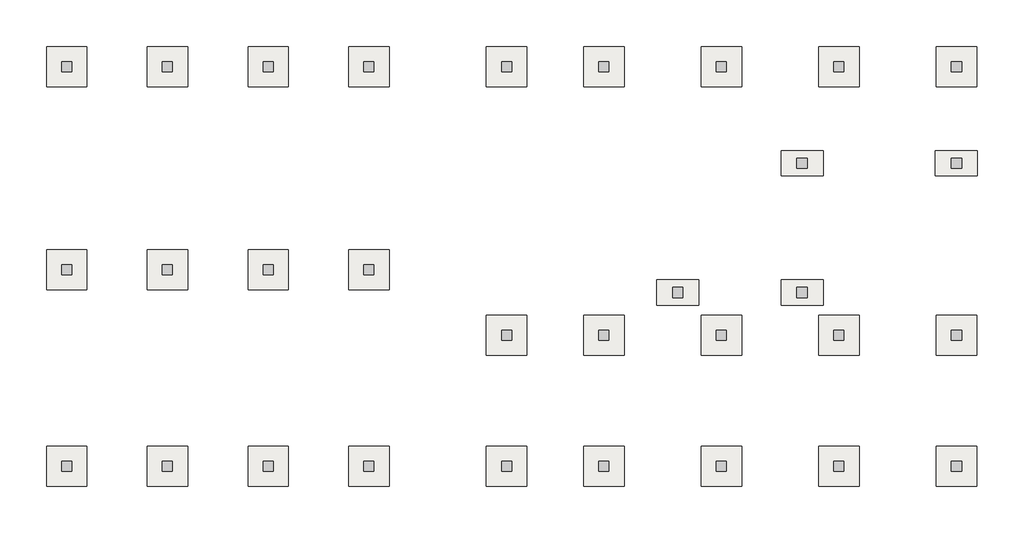
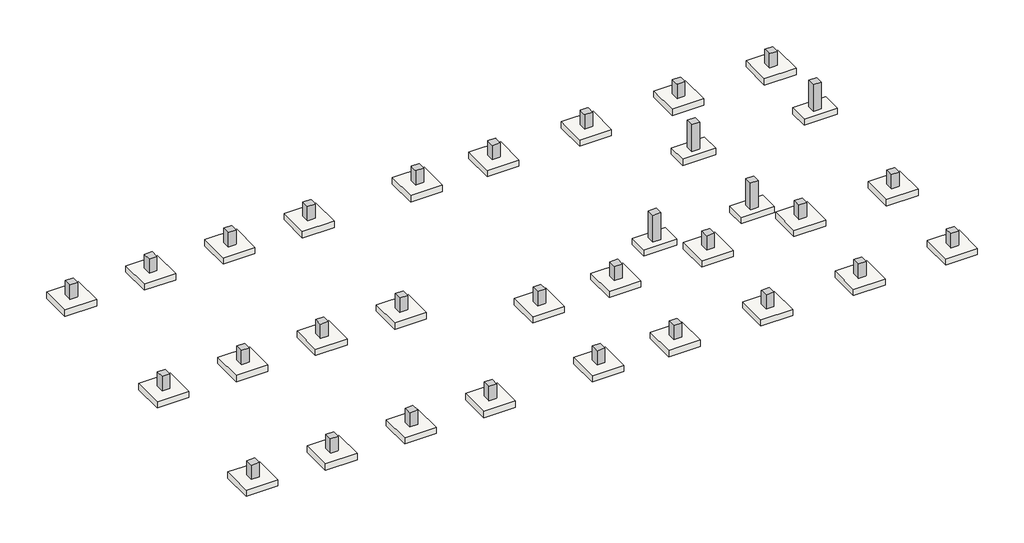
# Not in any storey: 31 columns, 31 slabs.
"""IFC4 building model written with IfcOpenShell, lengths in millimetres."""

import ifcopenshell
import ifcopenshell.guid

model = None  # the IFC model being written
_history = None  # IfcOwnerHistory: only IFC2X3 demands one
_inside = {}  # id of a spatial element -> (the spatial element, [elements in it])
_under = {}  # id of a project, library or spatial element -> (it, [spatial elements below it])
_declared = {}  # id of a project -> (the project, [libraries it declares])
_typed = {}  # id of a type object -> (the type object, [elements of that type])
_made_of = {}  # id of a material, layer set ... -> (it, [elements and type objects made of it])


def new_model(schema):
    """Start an empty IFC model of exactly this schema.

    Asked for "IFC4X3", IfcOpenShell would pick the latest addendum, in which some entities
    have other attributes; the version numbers below select the first issue.
    IFC2X3 requires an IfcOwnerHistory on every rooted entity: one is made here for all.
    """
    global model, _history
    if schema == "IFC4X3":
        model = ifcopenshell.file(schema_version=(4, 3, 0, 0))
    else:
        model = ifcopenshell.file(schema=schema)
    _inside.clear()
    _under.clear()
    _declared.clear()
    _typed.clear()
    _made_of.clear()
    _history = None
    if model.schema == "IFC2X3":
        org = make("IfcOrganization", Name="unknown")
        user = make(
            "IfcPersonAndOrganization",
            ThePerson=make("IfcPerson", FamilyName="unknown"),
            TheOrganization=org,
        )
        app = make(
            "IfcApplication",
            ApplicationDeveloper=org,
            Version="unknown",
            ApplicationFullName="unknown",
            ApplicationIdentifier="unknown",
        )
        _history = make(
            "IfcOwnerHistory",
            OwningUser=user,
            OwningApplication=app,
            ChangeAction="ADDED",
            CreationDate=0,
        )
    return model


def make(cls, **values):
    """One entity of the class cls with the attributes given. An attribute that is None is left unset."""
    return model.create_entity(
        cls, **{name: value for name, value in values.items() if value is not None}
    )


def rooted(cls, **values):
    """An entity with a GlobalId (a new one), such as an element, a storey or a relation."""
    return make(cls, GlobalId=ifcopenshell.guid.new(), OwnerHistory=_history, **values)


def si_unit(unit_type, name, prefix=None):
    """IfcSIUnit, for example si_unit("LENGTHUNIT", "METRE", prefix="MILLI")."""
    return make("IfcSIUnit", UnitType=unit_type, Prefix=prefix, Name=name)


def assignment(units):
    """IfcUnitAssignment: the units of a project."""
    return None if units is None else make("IfcUnitAssignment", Units=units)


def point(xyz):
    """IfcCartesianPoint."""
    return None if xyz is None else make("IfcCartesianPoint", Coordinates=xyz)


def direction(xyz):
    """IfcDirection."""
    return None if xyz is None else make("IfcDirection", DirectionRatios=xyz)


def frame(location, z_axis=None, x_axis=None):
    """IfcAxis2Placement3D, a coordinate frame: its origin and axes. An axis left out is left unset."""
    return make(
        "IfcAxis2Placement3D",
        Location=point(location),
        Axis=direction(z_axis),
        RefDirection=direction(x_axis),
    )


def origin():
    """The frame at (0, 0, 0) with its axes left unset."""
    return frame((0.0, 0.0, 0.0))


def place(relative_to, where):
    """IfcLocalPlacement: puts the frame where relative to a parent placement (None: the world)."""
    return make(
        "IfcLocalPlacement", PlacementRelTo=relative_to, RelativePlacement=where
    )


def context(
    kind, dimensions, precision=None, world=None, true_north=None, identifier=None
):
    """IfcGeometricRepresentationContext, for example the 3D "Model" context."""
    return make(
        "IfcGeometricRepresentationContext",
        ContextIdentifier=identifier,
        ContextType=kind,
        CoordinateSpaceDimension=dimensions,
        Precision=precision,
        WorldCoordinateSystem=world,
        TrueNorth=true_north,
    )


def project(units=None, contexts=None):
    """IfcProject with its units and contexts."""
    return rooted(
        "IfcProject",
        Name="project",
        RepresentationContexts=contexts,
        UnitsInContext=assignment(units),
    )


def spatial(cls, under=None, at=None, **own):
    """A site, building, storey or space (cls), placed at a placement, below another one or the project."""
    s = rooted(cls, ObjectPlacement=at, **own)
    if under is not None:
        _under.setdefault(under.id(), (under, []))[1].append(s)
    return s


def polyline(points):
    """IfcPolyline through the points."""
    return make("IfcPolyline", Points=[point(p) for p in points])


def outline(outer, holes=None, kind="AREA"):
    """IfcArbitraryClosedProfileDef: a profile drawn as a closed curve; with holes, ...WithVoids."""
    if holes is None:
        return make("IfcArbitraryClosedProfileDef", ProfileType=kind, OuterCurve=outer)
    return make(
        "IfcArbitraryProfileDefWithVoids",
        ProfileType=kind,
        OuterCurve=outer,
        InnerCurves=holes,
    )


def extrude(swept, where, along, depth):
    """IfcExtrudedAreaSolid: the profile swept, set in the frame where, extruded along a direction by depth."""
    return make(
        "IfcExtrudedAreaSolid",
        SweptArea=swept,
        Position=where,
        ExtrudedDirection=direction(along),
        Depth=depth,
    )


def faces_of(points, faces, orient=None, outer=None):
    """IfcFace entities. A face is a list of loops; a loop is a list of indices into points, from 0.

    orient and outer hold one flag for each loop. By default every Orientation is true, the
    first loop of a face is its IfcFaceOuterBound and the others are IfcFaceBound.
    """
    made = []
    for i, loops in enumerate(faces):
        bounds = []
        for j, loop in enumerate(loops):
            is_outer = j == 0 if outer is None else outer[i][j]
            bounds.append(
                make(
                    "IfcFaceOuterBound" if is_outer else "IfcFaceBound",
                    Bound=make("IfcPolyLoop", Polygon=[points[k] for k in loop]),
                    Orientation=True if orient is None else orient[i][j],
                )
            )
        made.append(make("IfcFace", Bounds=bounds))
    return made


def faceted_brep(points, faces, orient=None, outer=None, voids=None):
    """IfcFacetedBrep: a solid bounded by flat faces; with voids (closed shells), ...WithVoids."""
    shared = [point(p) for p in points]
    hull = make("IfcClosedShell", CfsFaces=faces_of(shared, faces, orient, outer))
    if voids is None:
        return make("IfcFacetedBrep", Outer=hull)
    return make(
        "IfcFacetedBrepWithVoids",
        Outer=hull,
        Voids=[
            make(cls, CfsFaces=faces_of(shared, fs, o, b)) for cls, fs, o, b in voids
        ],
    )


def shape(context_of_items, identifier, shape_type, items):
    """IfcShapeRepresentation: the items that make up one representation, for example the "Body"."""
    return make(
        "IfcShapeRepresentation",
        ContextOfItems=context_of_items,
        RepresentationIdentifier=identifier,
        RepresentationType=shape_type,
        Items=items,
    )


def source(mapping_origin, context_of_items, identifier, shape_type, items):
    """IfcRepresentationMap: a shape defined once, which mapped items show again and again."""
    return make(
        "IfcRepresentationMap",
        MappingOrigin=mapping_origin,
        MappedRepresentation=shape(context_of_items, identifier, shape_type, items),
    )


def transform(
    local_origin,
    x_axis=None,
    y_axis=None,
    z_axis=None,
    scale=None,
    scale2=None,
    scale3=None,
    uniform=True,
):
    """IfcCartesianTransformationOperator3D, or its non-uniform kind. x_axis, y_axis, z_axis: its Axis1, 2, 3."""
    if uniform:
        return make(
            "IfcCartesianTransformationOperator3D",
            Axis1=direction(x_axis),
            Axis2=direction(y_axis),
            LocalOrigin=point(local_origin),
            Scale=scale,
            Axis3=direction(z_axis),
        )
    return make(
        "IfcCartesianTransformationOperator3DnonUniform",
        Axis1=direction(x_axis),
        Axis2=direction(y_axis),
        LocalOrigin=point(local_origin),
        Scale=scale,
        Axis3=direction(z_axis),
        Scale2=scale2,
        Scale3=scale3,
    )


def mapped(mapping_source, mapping_target):
    """IfcMappedItem: shows the shape of a source again, moved by a transform."""
    return make(
        "IfcMappedItem", MappingSource=mapping_source, MappingTarget=mapping_target
    )


def made_of(thing, what):
    """Note that an element or type object is made of a material, layer set ...; save() writes the relation."""
    if what is not None:
        _made_of.setdefault(what.id(), (what, []))[1].append(thing)
    return thing


def element(
    cls,
    number,
    at=None,
    inside=None,
    cuts=None,
    type_object=None,
    material=None,
    context=None,
    identifier="Body",
    shape_type=None,
    held_by="IfcProductDefinitionShape",
    body=None,
    shapes=None,
    **own,
):
    """One element of the class cls, such as IfcWall. Its Tag is "e" and its number.

    at: its placement. inside: the storey or other place that contains it. cuts: it is an
    opening in that element (IfcRelVoidsElement). A single representation is given by context,
    identifier, shape_type and body (its items); several are given by shapes. held_by: the class
    of the entity that holds the representations. save() writes the other relations.
    """
    e = rooted(cls, Tag="e%d" % number, ObjectPlacement=at, **own)
    if body is not None:
        shapes = [shape(context, identifier, shape_type, body)]
    if shapes is not None:
        e.Representation = make(held_by, Representations=shapes)
    if inside is not None:
        _inside.setdefault(inside.id(), (inside, []))[1].append(e)
    if cuts is not None:
        rooted(
            "IfcRelVoidsElement", RelatingBuildingElement=cuts, RelatedOpeningElement=e
        )
    if type_object is not None:
        _typed.setdefault(type_object.id(), (type_object, []))[1].append(e)
    return made_of(e, material)


def aggregate(whole, parts):
    """IfcRelAggregates: a whole, such as a stair, and the parts it consists of."""
    return rooted("IfcRelAggregates", RelatingObject=whole, RelatedObjects=parts)


def save(model, path):
    """Write the relations noted so far, then the file.

    IfcRelAggregates (storeys below a building ...), IfcRelContainedInSpatialStructure (elements
    in a storey), IfcRelDefinesByType, IfcRelAssociatesMaterial and IfcRelDeclares: one each for
    every whole, place, type object, material and project.
    """
    for whole, parts in _under.values():
        aggregate(whole, parts)
    for where, things in _inside.values():
        rooted(
            "IfcRelContainedInSpatialStructure",
            RelatedElements=things,
            RelatingStructure=where,
        )
    for kind, things in _typed.values():
        rooted("IfcRelDefinesByType", RelatedObjects=things, RelatingType=kind)
    for what, things in _made_of.values():
        rooted("IfcRelAssociatesMaterial", RelatedObjects=things, RelatingMaterial=what)
    for by, libraries in _declared.values():
        rooted("IfcRelDeclares", RelatingContext=by, RelatedDefinitions=libraries)
    model.write(path)


def ft211_footing_rectangular_r1_5fe39465(model_context):
    return source(origin(), model_context, "Body", "SweptSolid", [
        extrude(outline(polyline([(1200.0, 1200.0), (1200.0, -1200.0), (-1200.0, -1200.0), (-1200.0, 1200.0), (1200.0, 1200.0)])), frame((0.0, 0.0, -500.0), z_axis=(0.0, 0.0, 1.0), x_axis=(1.0, 0.0, 0.0)), (0.0, 0.0, 1.0), 500.0),
    ])


def ft211_footing_rectangular_r1_907a7f09(model_context):
    return source(origin(), model_context, "Body", "SweptSolid", [
        extrude(outline(polyline([(1250.0, 750.0), (1250.0, -750.0), (-1250.0, -750.0), (-1250.0, 750.0), (1250.0, 750.0)])), frame((0.0, 0.0, -500.0), z_axis=(0.0, 0.0, 1.0), x_axis=(1.0, 0.0, 0.0)), (0.0, 0.0, 1.0), 500.0),
    ])


model = new_model("IFC4")

# Units and contexts
model_context = context("Model", 3, world=origin())
ifc_project = project(units=[si_unit("LENGTHUNIT", "METRE", prefix="MILLI")], contexts=[model_context])

# Site, building
site = spatial("IfcSite", under=ifc_project)
building = spatial("IfcBuilding", under=site)

# Columns
placement = place(None, origin())
element("IfcColumn", 1, ObjectType="RC_Column_Rectangular : H_SC_ACC_UG PED_W600xL600", at=placement, inside=building, context=model_context, shape_type="SweptSolid", body=[
    extrude(outline(polyline([(224.7, 12616.5208589), (224.7, 12016.5208589), (-375.3, 12016.5208589), (-375.3, 12616.5208589), (224.7, 12616.5208589)])), frame((0.0, 0.0, -1000.0), z_axis=(0.0, 0.0, 1.0), x_axis=(1.0, 0.0, 0.0)), (0.0, 0.0, 1.0), 1150.0),
])
element("IfcColumn", 2, ObjectType="RC_Column_Rectangular : H_SC_ACC_UG PED_W600xL600", at=placement, inside=building, context=model_context, shape_type="SweptSolid", body=[
    extrude(outline(polyline([(6224.7, 12616.5208589), (6224.7, 12016.5208589), (5624.7, 12016.5208589), (5624.7, 12616.5208589), (6224.7, 12616.5208589)])), frame((0.0, 0.0, -1000.0), z_axis=(0.0, 0.0, 1.0), x_axis=(1.0, 0.0, 0.0)), (0.0, 0.0, 1.0), 1150.0),
])
element("IfcColumn", 3, ObjectType="RC_Column_Rectangular : H_SC_ACC_UG PED_W600xL600", at=placement, inside=building, context=model_context, shape_type="SweptSolid", body=[
    extrude(outline(polyline([(12224.7, 12616.5208589), (12224.7, 12016.5208589), (11624.7, 12016.5208589), (11624.7, 12616.5208589), (12224.7, 12616.5208589)])), frame((0.0, 0.0, -1000.0), z_axis=(0.0, 0.0, 1.0), x_axis=(1.0, 0.0, 0.0)), (0.0, 0.0, 1.0), 1150.0),
])
element("IfcColumn", 4, ObjectType="RC_Column_Rectangular : H_SC_ACC_UG PED_W600xL600", at=placement, inside=building, context=model_context, shape_type="SweptSolid", body=[
    extrude(outline(polyline([(18224.7, 12616.5208589), (18224.7, 12016.5208589), (17624.7, 12016.5208589), (17624.7, 12616.5208589), (18224.7, 12616.5208589)])), frame((0.0, 0.0, -1000.0), z_axis=(0.0, 0.0, 1.0), x_axis=(1.0, 0.0, 0.0)), (0.0, 0.0, 1.0), 1150.0),
])
element("IfcColumn", 5, ObjectType="RC_Column_Rectangular : H_SC_ACC_UG PED_W600xL600", at=placement, inside=building, context=model_context, shape_type="SweptSolid", body=[
    extrude(outline(polyline([(224.7, 24716.5208589), (224.7, 24116.5208589), (-375.3, 24116.5208589), (-375.3, 24716.5208589), (224.7, 24716.5208589)])), frame((0.0, 0.0, -1000.0), z_axis=(0.0, 0.0, 1.0), x_axis=(1.0, 0.0, 0.0)), (0.0, 0.0, 1.0), 1150.0),
])
element("IfcColumn", 6, ObjectType="RC_Column_Rectangular : H_SC_ACC_UG PED_W600xL600", at=placement, inside=building, context=model_context, shape_type="SweptSolid", body=[
    extrude(outline(polyline([(6224.7, 24716.5208589), (6224.7, 24116.5208589), (5624.7, 24116.5208589), (5624.7, 24716.5208589), (6224.7, 24716.5208589)])), frame((0.0, 0.0, -1000.0), z_axis=(0.0, 0.0, 1.0), x_axis=(1.0, 0.0, 0.0)), (0.0, 0.0, 1.0), 1150.0),
])
element("IfcColumn", 7, ObjectType="RC_Column_Rectangular : H_SC_ACC_UG PED_W600xL600", at=placement, inside=building, context=model_context, shape_type="SweptSolid", body=[
    extrude(outline(polyline([(12224.7, 24716.5208589), (12224.7, 24116.5208589), (11624.7, 24116.5208589), (11624.7, 24716.5208589), (12224.7, 24716.5208589)])), frame((0.0, 0.0, -1000.0), z_axis=(0.0, 0.0, 1.0), x_axis=(1.0, 0.0, 0.0)), (0.0, 0.0, 1.0), 1150.0),
])
element("IfcColumn", 8, ObjectType="RC_Column_Rectangular : H_SC_ACC_UG PED_W600xL600", at=placement, inside=building, context=model_context, shape_type="Brep", body=[
    faceted_brep([(18224.7, 24716.5208589, -1000.0), (18224.7, 24116.5208589, -1000.0), (17624.7, 24116.5208589, -1000.0), (17624.7, 24716.5208589, -1000.0), (18224.7, 24716.5208589, 150.0), (18224.7, 24616.5208589, 150.0), (18224.7, 24216.5208589, 150.0), (18224.7, 24116.5208589, 150.0), (17624.7, 24116.5208589, 150.0), (17624.7, 24716.5208589, 150.0)], [[[0, 1, 2, 3]], [[4, 5, 6, 7, 1, 0]], [[7, 8, 2, 1]], [[8, 9, 3, 2]], [[9, 4, 0, 3]], [[4, 9, 8, 7, 6, 5]]]),
])
element("IfcColumn", 9, ObjectType="RC_Column_Rectangular : H_SC_ACC_UG PED_W600xL600", at=placement, inside=building, context=model_context, shape_type="Brep", body=[
    faceted_brep([(26424.7, 24716.5208589, -1000.0), (26424.7, 24116.5208589, -1000.0), (25824.7, 24116.5208589, -1000.0), (25824.7, 24716.5208589, -1000.0), (26424.7, 24716.5208589, 150.0), (26424.7, 24616.5208589, 150.0), (26424.7, 24216.5208589, 150.0), (26424.7, 24116.5208589, 150.0), (25824.7, 24116.5208589, 150.0), (25824.7, 24216.5208589, 150.0), (25824.7, 24616.5208589, 150.0), (25824.7, 24716.5208589, 150.0)], [[[0, 1, 2, 3]], [[4, 5, 6, 7, 1, 0]], [[7, 8, 2, 1]], [[8, 9, 10, 11, 3, 2]], [[11, 4, 0, 3]], [[4, 11, 10, 9, 8, 7, 6, 5]]]),
])
element("IfcColumn", 10, ObjectType="RC_Column_Rectangular : H_SC_ACC_UG PED_W600xL600", at=placement, inside=building, context=model_context, shape_type="Brep", body=[
    faceted_brep([(32224.7, 24716.5208589, -1000.0), (32224.7, 24116.5208589, -1000.0), (31624.7, 24116.5208589, -1000.0), (31624.7, 24716.5208589, -1000.0), (32224.7, 24716.5208589, 150.0), (32224.7, 24616.5208589, 150.0), (32224.7, 24216.5208589, 150.0), (32224.7, 24116.5208589, 150.0), (31624.7, 24116.5208589, 150.0), (31624.7, 24216.5208589, 150.0), (31624.7, 24616.5208589, 150.0), (31624.7, 24716.5208589, 150.0)], [[[0, 1, 2, 3]], [[4, 5, 6, 7, 1, 0]], [[7, 8, 2, 1]], [[8, 9, 10, 11, 3, 2]], [[11, 4, 0, 3]], [[4, 11, 10, 9, 8, 7, 6, 5]]]),
])
element("IfcColumn", 11, ObjectType="RC_Column_Rectangular : H_SC_ACC_UG PED_W600xL600", at=placement, inside=building, context=model_context, shape_type="Brep", body=[
    faceted_brep([(39224.7, 24716.5208589, -1000.0), (39224.7, 24116.5208589, -1000.0), (38624.7, 24116.5208589, -1000.0), (38624.7, 24716.5208589, -1000.0), (39224.7, 24716.5208589, 150.0), (39224.7, 24616.5208589, 150.0), (39224.7, 24216.5208589, 150.0), (39224.7, 24116.5208589, 150.0), (38624.7, 24116.5208589, 150.0), (38624.7, 24216.5208589, 150.0), (38624.7, 24616.5208589, 150.0), (38624.7, 24716.5208589, 150.0)], [[[0, 1, 2, 3]], [[4, 5, 6, 7, 1, 0]], [[7, 8, 2, 1]], [[8, 9, 10, 11, 3, 2]], [[11, 4, 0, 3]], [[4, 11, 10, 9, 8, 7, 6, 5]]]),
])
element("IfcColumn", 12, ObjectType="RC_Column_Rectangular : H_SC_ACC_UG PED_W600xL600", at=placement, inside=building, context=model_context, shape_type="Brep", body=[
    faceted_brep([(46224.7, 24716.5208589, -1000.0), (46224.7, 24116.5208589, -1000.0), (45624.7, 24116.5208589, -1000.0), (45624.7, 24716.5208589, -1000.0), (46224.7, 24716.5208589, 150.0), (46224.7, 24616.5208589, 150.0), (46224.7, 24216.5208589, 150.0), (46224.7, 24116.5208589, 150.0), (45624.7, 24116.5208589, 150.0), (45624.7, 24216.5208589, 150.0), (45624.7, 24616.5208589, 150.0), (45624.7, 24716.5208589, 150.0)], [[[0, 1, 2, 3]], [[4, 5, 6, 7, 1, 0]], [[7, 8, 2, 1]], [[8, 9, 10, 11, 3, 2]], [[11, 4, 0, 3]], [[4, 11, 10, 9, 8, 7, 6, 5]]]),
])
element("IfcColumn", 13, ObjectType="RC_Column_Rectangular : H_SC_ACC_UG PED_W600xL600", at=placement, inside=building, context=model_context, shape_type="Brep", body=[
    faceted_brep([(53224.7, 24716.5208589, -1000.0), (53224.7, 24116.5208589, -1000.0), (52624.7, 24116.5208589, -1000.0), (52624.7, 24716.5208589, -1000.0), (53224.7, 24716.5208589, 150.0), (53224.7, 24116.5208589, 150.0), (53124.7, 24116.5208589, 150.0), (52724.7, 24116.5208589, 150.0), (52624.7, 24116.5208589, 150.0), (52624.7, 24216.5208589, 150.0), (52624.7, 24616.5208589, 150.0), (52624.7, 24716.5208589, 150.0)], [[[0, 1, 2, 3]], [[4, 5, 1, 0]], [[5, 6, 7, 8, 2, 1]], [[8, 9, 10, 11, 3, 2]], [[11, 4, 0, 3]], [[4, 11, 10, 9, 8, 7, 6, 5]]]),
])
element("IfcColumn", 14, ObjectType="RC_Column_Rectangular : H_SC_ACC_UG PED_W600xL600", at=placement, inside=building, context=model_context, shape_type="SweptSolid", body=[
    extrude(outline(polyline([(26424.7, 8716.5208589), (26424.7, 8116.5208589), (25824.7, 8116.5208589), (25824.7, 8716.5208589), (26424.7, 8716.5208589)])), frame((0.0, 0.0, -1000.0), z_axis=(0.0, 0.0, 1.0), x_axis=(1.0, 0.0, 0.0)), (0.0, 0.0, 1.0), 1150.0),
])
element("IfcColumn", 15, ObjectType="RC_Column_Rectangular : H_SC_ACC_UG PED_W600xL600", at=placement, inside=building, context=model_context, shape_type="SweptSolid", body=[
    extrude(outline(polyline([(32224.7, 8716.5208589), (32224.7, 8116.5208589), (31624.7, 8116.5208589), (31624.7, 8716.5208589), (32224.7, 8716.5208589)])), frame((0.0, 0.0, -1000.0), z_axis=(0.0, 0.0, 1.0), x_axis=(1.0, 0.0, 0.0)), (0.0, 0.0, 1.0), 1150.0),
])
element("IfcColumn", 16, ObjectType="RC_Column_Rectangular : H_SC_ACC_UG PED_W600xL600", at=placement, inside=building, context=model_context, shape_type="SweptSolid", body=[
    extrude(outline(polyline([(39224.7, 8716.5208589), (39224.7, 8116.5208589), (38624.7, 8116.5208589), (38624.7, 8716.5208589), (39224.7, 8716.5208589)])), frame((0.0, 0.0, -1000.0), z_axis=(0.0, 0.0, 1.0), x_axis=(1.0, 0.0, 0.0)), (0.0, 0.0, 1.0), 1150.0),
])
element("IfcColumn", 17, ObjectType="RC_Column_Rectangular : H_SC_ACC_UG PED_W600xL600", at=placement, inside=building, context=model_context, shape_type="SweptSolid", body=[
    extrude(outline(polyline([(46224.7, 8716.5208589), (46224.7, 8116.5208589), (45624.7, 8116.5208589), (45624.7, 8716.5208589), (46224.7, 8716.5208589)])), frame((0.0, 0.0, -1000.0), z_axis=(0.0, 0.0, 1.0), x_axis=(1.0, 0.0, 0.0)), (0.0, 0.0, 1.0), 1150.0),
])
element("IfcColumn", 18, ObjectType="RC_Column_Rectangular : H_SC_ACC_UG PED_W600xL600", at=placement, inside=building, context=model_context, shape_type="Brep", body=[
    faceted_brep([(53224.7, 8716.5208589, -1000.0), (53224.7, 8116.5208589, -1000.0), (52624.7, 8116.5208589, -1000.0), (52624.7, 8716.5208589, -1000.0), (53224.7, 8716.5208589, 150.0), (53224.7, 8116.5208589, 150.0), (53124.7, 8116.5208589, 150.0), (52724.7, 8116.5208589, 150.0), (52624.7, 8116.5208589, 150.0), (52624.7, 8716.5208589, 150.0), (52724.7, 8716.5208589, 150.0), (53124.7, 8716.5208589, 150.0)], [[[0, 1, 2, 3]], [[4, 5, 1, 0]], [[5, 6, 7, 8, 2, 1]], [[8, 9, 3, 2]], [[9, 10, 11, 4, 0, 3]], [[4, 11, 10, 9, 8, 7, 6, 5]]]),
])
element("IfcColumn", 19, ObjectType="RC_Column_Rectangular : H_SC_ACC_UG PED_W600xL600", at=placement, inside=building, context=model_context, shape_type="SweptSolid", body=[
    extrude(outline(polyline([(224.7, 916.5208589), (224.7, 316.5208589), (-375.3, 316.5208589), (-375.3, 916.5208589), (224.7, 916.5208589)])), frame((0.0, 0.0, -1000.0), z_axis=(0.0, 0.0, 1.0), x_axis=(1.0, 0.0, 0.0)), (0.0, 0.0, 1.0), 1150.0),
])
element("IfcColumn", 20, ObjectType="RC_Column_Rectangular : H_SC_ACC_UG PED_W600xL600", at=placement, inside=building, context=model_context, shape_type="SweptSolid", body=[
    extrude(outline(polyline([(6224.7, 916.5208589), (6224.7, 316.5208589), (5624.7, 316.5208589), (5624.7, 916.5208589), (6224.7, 916.5208589)])), frame((0.0, 0.0, -1000.0), z_axis=(0.0, 0.0, 1.0), x_axis=(1.0, 0.0, 0.0)), (0.0, 0.0, 1.0), 1150.0),
])
element("IfcColumn", 21, ObjectType="RC_Column_Rectangular : H_SC_ACC_UG PED_W600xL600", at=placement, inside=building, context=model_context, shape_type="SweptSolid", body=[
    extrude(outline(polyline([(12224.7, 916.5208589), (12224.7, 316.5208589), (11624.7, 316.5208589), (11624.7, 916.5208589), (12224.7, 916.5208589)])), frame((0.0, 0.0, -1000.0), z_axis=(0.0, 0.0, 1.0), x_axis=(1.0, 0.0, 0.0)), (0.0, 0.0, 1.0), 1150.0),
])
element("IfcColumn", 22, ObjectType="RC_Column_Rectangular : H_SC_ACC_UG PED_W600xL600", at=placement, inside=building, context=model_context, shape_type="Brep", body=[
    faceted_brep([(18224.7, 916.5208589, -1000.0), (18224.7, 316.5208589, -1000.0), (17624.7, 316.5208589, -1000.0), (17624.7, 916.5208589, -1000.0), (18224.7, 916.5208589, 150.0), (18224.7, 816.5208589, 150.0), (18224.7, 416.5208589, 150.0), (18224.7, 316.5208589, 150.0), (17624.7, 316.5208589, 150.0), (17624.7, 916.5208589, 150.0)], [[[0, 1, 2, 3]], [[4, 5, 6, 7, 1, 0]], [[7, 8, 2, 1]], [[8, 9, 3, 2]], [[9, 4, 0, 3]], [[4, 9, 8, 7, 6, 5]]]),
])
element("IfcColumn", 23, ObjectType="RC_Column_Rectangular : H_SC_ACC_UG PED_W600xL600", at=placement, inside=building, context=model_context, shape_type="Brep", body=[
    faceted_brep([(26424.7, 916.5208589, -1000.0), (26424.7, 316.5208589, -1000.0), (25824.7, 316.5208589, -1000.0), (25824.7, 916.5208589, -1000.0), (26424.7, 916.5208589, 150.0), (26424.7, 816.5208589, 150.0), (26424.7, 416.5208589, 150.0), (26424.7, 316.5208589, 150.0), (25824.7, 316.5208589, 150.0), (25824.7, 416.5208589, 150.0), (25824.7, 816.5208589, 150.0), (25824.7, 916.5208589, 150.0)], [[[0, 1, 2, 3]], [[4, 5, 6, 7, 1, 0]], [[7, 8, 2, 1]], [[8, 9, 10, 11, 3, 2]], [[11, 4, 0, 3]], [[4, 11, 10, 9, 8, 7, 6, 5]]]),
])
element("IfcColumn", 24, ObjectType="RC_Column_Rectangular : H_SC_ACC_UG PED_W600xL600", at=placement, inside=building, context=model_context, shape_type="Brep", body=[
    faceted_brep([(32224.7, 916.5208589, -1000.0), (32224.7, 316.5208589, -1000.0), (31624.7, 316.5208589, -1000.0), (31624.7, 916.5208589, -1000.0), (32224.7, 916.5208589, 150.0), (32224.7, 816.5208589, 150.0), (32224.7, 416.5208589, 150.0), (32224.7, 316.5208589, 150.0), (31624.7, 316.5208589, 150.0), (31624.7, 416.5208589, 150.0), (31624.7, 816.5208589, 150.0), (31624.7, 916.5208589, 150.0)], [[[0, 1, 2, 3]], [[4, 5, 6, 7, 1, 0]], [[7, 8, 2, 1]], [[8, 9, 10, 11, 3, 2]], [[11, 4, 0, 3]], [[4, 11, 10, 9, 8, 7, 6, 5]]]),
])
element("IfcColumn", 25, ObjectType="RC_Column_Rectangular : H_SC_ACC_UG PED_W600xL600", at=placement, inside=building, context=model_context, shape_type="Brep", body=[
    faceted_brep([(39224.7, 916.5208589, -1000.0), (39224.7, 316.5208589, -1000.0), (38624.7, 316.5208589, -1000.0), (38624.7, 916.5208589, -1000.0), (39224.7, 916.5208589, 150.0), (39224.7, 816.5208589, 150.0), (39224.7, 416.5208589, 150.0), (39224.7, 316.5208589, 150.0), (38624.7, 316.5208589, 150.0), (38624.7, 416.5208589, 150.0), (38624.7, 816.5208589, 150.0), (38624.7, 916.5208589, 150.0)], [[[0, 1, 2, 3]], [[4, 5, 6, 7, 1, 0]], [[7, 8, 2, 1]], [[8, 9, 10, 11, 3, 2]], [[11, 4, 0, 3]], [[4, 11, 10, 9, 8, 7, 6, 5]]]),
])
element("IfcColumn", 26, ObjectType="RC_Column_Rectangular : H_SC_ACC_UG PED_W600xL600", at=placement, inside=building, context=model_context, shape_type="Brep", body=[
    faceted_brep([(46224.7, 916.5208589, -1000.0), (46224.7, 316.5208589, -1000.0), (45624.7, 316.5208589, -1000.0), (45624.7, 916.5208589, -1000.0), (46224.7, 916.5208589, 150.0), (46224.7, 816.5208589, 150.0), (46224.7, 416.5208589, 150.0), (46224.7, 316.5208589, 150.0), (45624.7, 316.5208589, 150.0), (45624.7, 416.5208589, 150.0), (45624.7, 816.5208589, 150.0), (45624.7, 916.5208589, 150.0)], [[[0, 1, 2, 3]], [[4, 5, 6, 7, 1, 0]], [[7, 8, 2, 1]], [[8, 9, 10, 11, 3, 2]], [[11, 4, 0, 3]], [[4, 11, 10, 9, 8, 7, 6, 5]]]),
])
element("IfcColumn", 27, ObjectType="RC_Column_Rectangular : H_SC_ACC_UG PED_W600xL600", at=placement, inside=building, context=model_context, shape_type="Brep", body=[
    faceted_brep([(53224.7, 916.5208589, -1000.0), (53224.7, 316.5208589, -1000.0), (52624.7, 316.5208589, -1000.0), (52624.7, 916.5208589, -1000.0), (53224.7, 916.5208589, 150.0), (53224.7, 316.5208589, 150.0), (52624.7, 316.5208589, 150.0), (52624.7, 416.5208589, 150.0), (52624.7, 816.5208589, 150.0), (52624.7, 916.5208589, 150.0), (52724.7, 916.5208589, 150.0), (53124.7, 916.5208589, 150.0)], [[[0, 1, 2, 3]], [[4, 5, 1, 0]], [[5, 6, 2, 1]], [[6, 7, 8, 9, 3, 2]], [[9, 10, 11, 4, 0, 3]], [[4, 11, 10, 9, 8, 7, 6, 5]]]),
])
element("IfcColumn", 28, ObjectType="RC_Column_Rectangular : H_SC_ACC_UG PED_W600xL600", at=placement, inside=building, context=model_context, shape_type="SweptSolid", body=[
    extrude(outline(polyline([(36624.7, 11266.5208589), (36624.7, 10666.5208589), (36024.7, 10666.5208589), (36024.7, 11266.5208589), (36624.7, 11266.5208589)])), frame((0.0, 0.0, -1000.0), z_axis=(0.0, 0.0, 1.0), x_axis=(1.0, 0.0, 0.0)), (0.0, 0.0, 1.0), 2150.0),
])
element("IfcColumn", 29, ObjectType="RC_Column_Rectangular : H_SC_ACC_UG PED_W600xL600", at=placement, inside=building, context=model_context, shape_type="SweptSolid", body=[
    extrude(outline(polyline([(44024.7, 11266.5208589), (44024.7, 10666.5208589), (43424.7, 10666.5208589), (43424.7, 11266.5208589), (44024.7, 11266.5208589)])), frame((0.0, 0.0, -1000.0), z_axis=(0.0, 0.0, 1.0), x_axis=(1.0, 0.0, 0.0)), (0.0, 0.0, 1.0), 2150.0),
])
element("IfcColumn", 30, ObjectType="RC_Column_Rectangular : H_SC_ACC_UG PED_W600xL600", at=placement, inside=building, context=model_context, shape_type="SweptSolid", body=[
    extrude(outline(polyline([(44024.7, 18966.5208589), (44024.7, 18366.5208589), (43424.7, 18366.5208589), (43424.7, 18966.5208589), (44024.7, 18966.5208589)])), frame((0.0, 0.0, -1000.0), z_axis=(0.0, 0.0, 1.0), x_axis=(1.0, 0.0, 0.0)), (0.0, 0.0, 1.0), 2150.0),
])
element("IfcColumn", 31, ObjectType="RC_Column_Rectangular : H_SC_ACC_UG PED_W600xL600", at=placement, inside=building, context=model_context, shape_type="SweptSolid", body=[
    extrude(outline(polyline([(53224.7, 18966.5208589), (53224.7, 18366.5208589), (52624.7, 18366.5208589), (52624.7, 18966.5208589), (53224.7, 18966.5208589)])), frame((0.0, 0.0, -1000.0), z_axis=(0.0, 0.0, 1.0), x_axis=(1.0, 0.0, 0.0)), (0.0, 0.0, 1.0), 2150.0),
])

# Slabs
ft211_footing_rectangular_r1_shape = ft211_footing_rectangular_r1_5fe39465(model_context)
element("IfcSlab", 32, ObjectType="FT211-Footing-Rectangular_R1 : H_SF_ACF_W2400xL2400xT500_Bitumen", at=placement, inside=building, context=model_context, shape_type="MappedRepresentation", body=[
    mapped(ft211_footing_rectangular_r1_shape, transform((-75.3, 12316.5208589, -1000.0), x_axis=(1.0, 0.0, 0.0), y_axis=(0.0, 1.0, 0.0), z_axis=(0.0, 0.0, 1.0))),
])
element("IfcSlab", 33, ObjectType="FT211-Footing-Rectangular_R1 : H_SF_ACF_W2400xL2400xT500_Bitumen", at=placement, inside=building, context=model_context, shape_type="MappedRepresentation", body=[
    mapped(ft211_footing_rectangular_r1_shape, transform((5924.7, 12316.5208589, -1000.0), x_axis=(1.0, 0.0, 0.0), y_axis=(0.0, 1.0, 0.0), z_axis=(0.0, 0.0, 1.0))),
])
element("IfcSlab", 34, ObjectType="FT211-Footing-Rectangular_R1 : H_SF_ACF_W2400xL2400xT500_Bitumen", at=placement, inside=building, context=model_context, shape_type="MappedRepresentation", body=[
    mapped(ft211_footing_rectangular_r1_shape, transform((11924.7, 12316.5208589, -1000.0), x_axis=(1.0, 0.0, 0.0), y_axis=(0.0, 1.0, 0.0), z_axis=(0.0, 0.0, 1.0))),
])
element("IfcSlab", 35, ObjectType="FT211-Footing-Rectangular_R1 : H_SF_ACF_W2400xL2400xT500_Bitumen", at=placement, inside=building, context=model_context, shape_type="MappedRepresentation", body=[
    mapped(ft211_footing_rectangular_r1_shape, transform((17924.7, 12316.5208589, -1000.0), x_axis=(1.0, 0.0, 0.0), y_axis=(0.0, 1.0, 0.0), z_axis=(0.0, 0.0, 1.0))),
])
element("IfcSlab", 36, ObjectType="FT211-Footing-Rectangular_R1 : H_SF_ACF_W2400xL2400xT500_Bitumen", at=placement, inside=building, context=model_context, shape_type="MappedRepresentation", body=[
    mapped(ft211_footing_rectangular_r1_shape, transform((-75.3, 24416.5208589, -1000.0), x_axis=(1.0, 0.0, 0.0), y_axis=(0.0, 1.0, 0.0), z_axis=(0.0, 0.0, 1.0))),
])
element("IfcSlab", 37, ObjectType="FT211-Footing-Rectangular_R1 : H_SF_ACF_W2400xL2400xT500_Bitumen", at=placement, inside=building, context=model_context, shape_type="MappedRepresentation", body=[
    mapped(ft211_footing_rectangular_r1_shape, transform((5924.7, 24416.5208589, -1000.0), x_axis=(1.0, 0.0, 0.0), y_axis=(0.0, 1.0, 0.0), z_axis=(0.0, 0.0, 1.0))),
])
element("IfcSlab", 38, ObjectType="FT211-Footing-Rectangular_R1 : H_SF_ACF_W2400xL2400xT500_Bitumen", at=placement, inside=building, context=model_context, shape_type="MappedRepresentation", body=[
    mapped(ft211_footing_rectangular_r1_shape, transform((11924.7, 24416.5208589, -1000.0), x_axis=(1.0, 0.0, 0.0), y_axis=(0.0, 1.0, 0.0), z_axis=(0.0, 0.0, 1.0))),
])
element("IfcSlab", 39, ObjectType="FT211-Footing-Rectangular_R1 : H_SF_ACF_W2400xL2400xT500_Bitumen", at=placement, inside=building, context=model_context, shape_type="MappedRepresentation", body=[
    mapped(ft211_footing_rectangular_r1_shape, transform((17924.7, 24416.5208589, -1000.0), x_axis=(1.0, 0.0, 0.0), y_axis=(0.0, 1.0, 0.0), z_axis=(0.0, 0.0, 1.0))),
])
element("IfcSlab", 40, ObjectType="FT211-Footing-Rectangular_R1 : H_SF_ACF_W2400xL2400xT500_Bitumen", at=placement, inside=building, context=model_context, shape_type="MappedRepresentation", body=[
    mapped(ft211_footing_rectangular_r1_shape, transform((26124.7, 24416.5208589, -1000.0), x_axis=(1.0, 0.0, 0.0), y_axis=(0.0, 1.0, 0.0), z_axis=(0.0, 0.0, 1.0))),
])
element("IfcSlab", 41, ObjectType="FT211-Footing-Rectangular_R1 : H_SF_ACF_W2400xL2400xT500_Bitumen", at=placement, inside=building, context=model_context, shape_type="MappedRepresentation", body=[
    mapped(ft211_footing_rectangular_r1_shape, transform((31924.7, 24416.5208589, -1000.0), x_axis=(1.0, 0.0, 0.0), y_axis=(0.0, 1.0, 0.0), z_axis=(0.0, 0.0, 1.0))),
])
element("IfcSlab", 42, ObjectType="FT211-Footing-Rectangular_R1 : H_SF_ACF_W2400xL2400xT500_Bitumen", at=placement, inside=building, context=model_context, shape_type="MappedRepresentation", body=[
    mapped(ft211_footing_rectangular_r1_shape, transform((38924.7, 24416.5208589, -1000.0), x_axis=(1.0, 0.0, 0.0), y_axis=(0.0, 1.0, 0.0), z_axis=(0.0, 0.0, 1.0))),
])
element("IfcSlab", 43, ObjectType="FT211-Footing-Rectangular_R1 : H_SF_ACF_W2400xL2400xT500_Bitumen", at=placement, inside=building, context=model_context, shape_type="MappedRepresentation", body=[
    mapped(ft211_footing_rectangular_r1_shape, transform((45924.7, 24416.5208589, -1000.0), x_axis=(1.0, 0.0, 0.0), y_axis=(0.0, 1.0, 0.0), z_axis=(0.0, 0.0, 1.0))),
])
element("IfcSlab", 44, ObjectType="FT211-Footing-Rectangular_R1 : H_SF_ACF_W2400xL2400xT500_Bitumen", at=placement, inside=building, context=model_context, shape_type="MappedRepresentation", body=[
    mapped(ft211_footing_rectangular_r1_shape, transform((52924.7, 24416.5208589, -1000.0), x_axis=(1.0, 0.0, 0.0), y_axis=(0.0, 1.0, 0.0), z_axis=(0.0, 0.0, 1.0))),
])
element("IfcSlab", 45, ObjectType="FT211-Footing-Rectangular_R1 : H_SF_ACF_W2400xL2400xT500_Bitumen", at=placement, inside=building, context=model_context, shape_type="MappedRepresentation", body=[
    mapped(ft211_footing_rectangular_r1_shape, transform((26124.7, 8416.5208589, -1000.0), x_axis=(1.0, 0.0, 0.0), y_axis=(0.0, 1.0, 0.0), z_axis=(0.0, 0.0, 1.0))),
])
element("IfcSlab", 46, ObjectType="FT211-Footing-Rectangular_R1 : H_SF_ACF_W2400xL2400xT500_Bitumen", at=placement, inside=building, context=model_context, shape_type="MappedRepresentation", body=[
    mapped(ft211_footing_rectangular_r1_shape, transform((31924.7, 8416.5208589, -1000.0), x_axis=(1.0, 0.0, 0.0), y_axis=(0.0, 1.0, 0.0), z_axis=(0.0, 0.0, 1.0))),
])
element("IfcSlab", 47, ObjectType="FT211-Footing-Rectangular_R1 : H_SF_ACF_W2400xL2400xT500_Bitumen", at=placement, inside=building, context=model_context, shape_type="MappedRepresentation", body=[
    mapped(ft211_footing_rectangular_r1_shape, transform((38924.7, 8416.5208589, -1000.0), x_axis=(1.0, 0.0, 0.0), y_axis=(0.0, 1.0, 0.0), z_axis=(0.0, 0.0, 1.0))),
])
element("IfcSlab", 48, ObjectType="FT211-Footing-Rectangular_R1 : H_SF_ACF_W2400xL2400xT500_Bitumen", at=placement, inside=building, context=model_context, shape_type="MappedRepresentation", body=[
    mapped(ft211_footing_rectangular_r1_shape, transform((45924.7, 8416.5208589, -1000.0), x_axis=(1.0, 0.0, 0.0), y_axis=(0.0, 1.0, 0.0), z_axis=(0.0, 0.0, 1.0))),
])
element("IfcSlab", 49, ObjectType="FT211-Footing-Rectangular_R1 : H_SF_ACF_W2400xL2400xT500_Bitumen", at=placement, inside=building, context=model_context, shape_type="MappedRepresentation", body=[
    mapped(ft211_footing_rectangular_r1_shape, transform((52924.7, 8416.5208589, -1000.0), x_axis=(1.0, 0.0, 0.0), y_axis=(0.0, 1.0, 0.0), z_axis=(0.0, 0.0, 1.0))),
])
element("IfcSlab", 50, ObjectType="FT211-Footing-Rectangular_R1 : H_SF_ACF_W2400xL2400xT500_Bitumen", at=placement, inside=building, context=model_context, shape_type="MappedRepresentation", body=[
    mapped(ft211_footing_rectangular_r1_shape, transform((-75.3, 616.5208589, -1000.0), x_axis=(1.0, 0.0, 0.0), y_axis=(0.0, 1.0, 0.0), z_axis=(0.0, 0.0, 1.0))),
])
element("IfcSlab", 51, ObjectType="FT211-Footing-Rectangular_R1 : H_SF_ACF_W2400xL2400xT500_Bitumen", at=placement, inside=building, context=model_context, shape_type="MappedRepresentation", body=[
    mapped(ft211_footing_rectangular_r1_shape, transform((5924.7, 616.5208589, -1000.0), x_axis=(1.0, 0.0, 0.0), y_axis=(0.0, 1.0, 0.0), z_axis=(0.0, 0.0, 1.0))),
])
element("IfcSlab", 52, ObjectType="FT211-Footing-Rectangular_R1 : H_SF_ACF_W2400xL2400xT500_Bitumen", at=placement, inside=building, context=model_context, shape_type="MappedRepresentation", body=[
    mapped(ft211_footing_rectangular_r1_shape, transform((11924.7, 616.5208589, -1000.0), x_axis=(1.0, 0.0, 0.0), y_axis=(0.0, 1.0, 0.0), z_axis=(0.0, 0.0, 1.0))),
])
element("IfcSlab", 53, ObjectType="FT211-Footing-Rectangular_R1 : H_SF_ACF_W2400xL2400xT500_Bitumen", at=placement, inside=building, context=model_context, shape_type="MappedRepresentation", body=[
    mapped(ft211_footing_rectangular_r1_shape, transform((17924.7, 616.5208589, -1000.0), x_axis=(1.0, 0.0, 0.0), y_axis=(0.0, 1.0, 0.0), z_axis=(0.0, 0.0, 1.0))),
])
element("IfcSlab", 54, ObjectType="FT211-Footing-Rectangular_R1 : H_SF_ACF_W2400xL2400xT500_Bitumen", at=placement, inside=building, context=model_context, shape_type="MappedRepresentation", body=[
    mapped(ft211_footing_rectangular_r1_shape, transform((26124.7, 616.5208589, -1000.0), x_axis=(1.0, 0.0, 0.0), y_axis=(0.0, 1.0, 0.0), z_axis=(0.0, 0.0, 1.0))),
])
element("IfcSlab", 55, ObjectType="FT211-Footing-Rectangular_R1 : H_SF_ACF_W2400xL2400xT500_Bitumen", at=placement, inside=building, context=model_context, shape_type="MappedRepresentation", body=[
    mapped(ft211_footing_rectangular_r1_shape, transform((31924.7, 616.5208589, -1000.0), x_axis=(1.0, 0.0, 0.0), y_axis=(0.0, 1.0, 0.0), z_axis=(0.0, 0.0, 1.0))),
])
element("IfcSlab", 56, ObjectType="FT211-Footing-Rectangular_R1 : H_SF_ACF_W2400xL2400xT500_Bitumen", at=placement, inside=building, context=model_context, shape_type="MappedRepresentation", body=[
    mapped(ft211_footing_rectangular_r1_shape, transform((38924.7, 616.5208589, -1000.0), x_axis=(1.0, 0.0, 0.0), y_axis=(0.0, 1.0, 0.0), z_axis=(0.0, 0.0, 1.0))),
])
element("IfcSlab", 57, ObjectType="FT211-Footing-Rectangular_R1 : H_SF_ACF_W2400xL2400xT500_Bitumen", at=placement, inside=building, context=model_context, shape_type="MappedRepresentation", body=[
    mapped(ft211_footing_rectangular_r1_shape, transform((45924.7, 616.5208589, -1000.0), x_axis=(1.0, 0.0, 0.0), y_axis=(0.0, 1.0, 0.0), z_axis=(0.0, 0.0, 1.0))),
])
element("IfcSlab", 58, ObjectType="FT211-Footing-Rectangular_R1 : H_SF_ACF_W2400xL2400xT500_Bitumen", at=placement, inside=building, context=model_context, shape_type="MappedRepresentation", body=[
    mapped(ft211_footing_rectangular_r1_shape, transform((52924.7, 616.5208589, -1000.0), x_axis=(1.0, 0.0, 0.0), y_axis=(0.0, 1.0, 0.0), z_axis=(0.0, 0.0, 1.0))),
])
ft211_footing_rectangular_r1_2_shape = ft211_footing_rectangular_r1_907a7f09(model_context)
element("IfcSlab", 59, ObjectType="FT211-Footing-Rectangular_R1 : H_SF_ACF_W2500xL1500xT500_Bitumen", at=placement, inside=building, context=model_context, shape_type="MappedRepresentation", body=[
    mapped(ft211_footing_rectangular_r1_2_shape, transform((36324.7, 10966.5208589, -1000.0), x_axis=(1.0, 0.0, 0.0), y_axis=(0.0, 1.0, 0.0), z_axis=(0.0, 0.0, 1.0))),
])
element("IfcSlab", 60, ObjectType="FT211-Footing-Rectangular_R1 : H_SF_ACF_W2500xL1500xT500_Bitumen", at=placement, inside=building, context=model_context, shape_type="MappedRepresentation", body=[
    mapped(ft211_footing_rectangular_r1_2_shape, transform((43724.7, 10966.5208589, -1000.0), x_axis=(1.0, 0.0, 0.0), y_axis=(0.0, 1.0, 0.0), z_axis=(0.0, 0.0, 1.0))),
])
element("IfcSlab", 61, ObjectType="FT211-Footing-Rectangular_R1 : H_SF_ACF_W2500xL1500xT500_Bitumen", at=placement, inside=building, context=model_context, shape_type="MappedRepresentation", body=[
    mapped(ft211_footing_rectangular_r1_2_shape, transform((43724.7, 18666.5208589, -1000.0), x_axis=(1.0, 0.0, 0.0), y_axis=(0.0, 1.0, 0.0), z_axis=(0.0, 0.0, 1.0))),
])
element("IfcSlab", 62, ObjectType="FT211-Footing-Rectangular_R1 : H_SF_ACF_W2500xL1500xT500_Bitumen", at=placement, inside=building, context=model_context, shape_type="MappedRepresentation", body=[
    mapped(ft211_footing_rectangular_r1_2_shape, transform((52924.7, 18666.5208589, -1000.0), x_axis=(1.0, 0.0, 0.0), y_axis=(0.0, 1.0, 0.0), z_axis=(0.0, 0.0, 1.0))),
])

save(model, "model.ifc")

# Revit data of these elements
# Type "RC_Column_Rectangular : H_SC_ACC_UG PED_W600xL600"
#   Width = 600.000 mm
#   Length = 600.000 mm
#   hec_material3 [instance default] = none
#   hec_material2 [instance default] = none
#   hec_material1 [instance default] = none
#   Structural Material [instance default] = none
#   Description = (empty or 0)
# Type "FT211-Footing-Rectangular_R1 : H_SF_ACF_W2400xL2400xT500_Bitumen"
#   Top bar = "D25@300"
#   Description = "UG Shallow Foundation"
#   Bottom bar = "D20@300"
#   Width = 2400.000 mm
#   Length = 2400.000 mm
#   Foundation Thickness = 500.000 mm
#   Structural Material [instance default] = none
#   Assembly Code = ""
# Type "FT211-Footing-Rectangular_R1 : H_SF_ACF_W2500xL1500xT500_Bitumen"
#   Top bar = "D25@300"
#   Description = "UG Shallow Foundation"
#   Bottom bar = "D20@300"
#   Width = 2500.000 mm
#   Length = 1500.000 mm
#   Foundation Thickness = 500.000 mm
#   Structural Material [instance default] = none
#   Assembly Code = ""
# Elements 1, 2, 3, 4, 5, 6, 7, 8, 9, 10, 11, 12, 13, 14, 15, 16, 17, 18, 19, 20, 21, 22, 23, 24, 25, 26, 27, 28, 29, 30, 31 (IfcColumn, "RC_Column_Rectangular : H_SC_ACC_UG PED_W600xL600")
#   Comments = ""
#   hec_material3 = none
#   hec_material2 = none
#   hec_material1 = none
#   Structural Material = none
#   Phase Created = New Construction
# Elements 32, 33, 34, 35, 36, 37, 38, 39, 40, 41, 42, 43, 44, 45, 46, 47, 48, 49, 50, 51, 52, 53, 54, 55, 56, 57, 58 (IfcSlab, "FT211-Footing-Rectangular_R1 : H_SF_ACF_W2400xL2400xT500_Bitumen")
#   Comments = ""
#   Structural Material = none
#   Phase Created = New Construction
# Elements 59, 60, 61, 62 (IfcSlab, "FT211-Footing-Rectangular_R1 : H_SF_ACF_W2500xL1500xT500_Bitumen")
#   Comments = ""
#   Structural Material = none
#   Phase Created = New Construction
